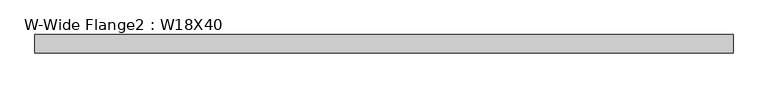
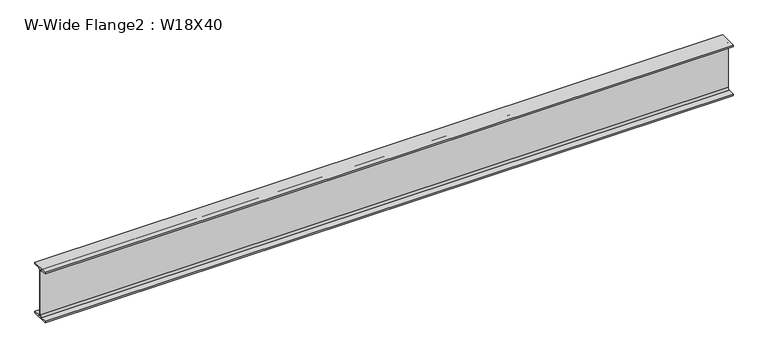
"""IFC4 building model written with IfcOpenShell, lengths in millimetres: beam geometry, W-Wide Flange2 : W18X40."""

from ifc_helpers import new_model, si_unit, point, frame, frame_2d, origin, place, context, project, spatial, polyline, circle_curve, trimmed, segment, composite_curve, outline, extrude, source, transform, mapped, element, save


def w_wide_flange2_w18x40_2cca02ce(model_context):
    return source(origin(), model_context, "Body", "SweptSolid", [
        extrude(outline(composite_curve([segment(polyline([(76.454, -213.995), (76.454, -227.33), (-76.454, -227.33), (-76.454, -213.995), (-20.828, -213.995)]), True, "CONTINUOUS"), segment(trimmed(circle_curve(frame_2d((-20.828, -197.1675)), 16.8275), [point((-20.828, -213.995))], [point((-4.0005, -197.1675))], True, "CARTESIAN"), True, "CONTINUOUS"), segment(polyline([(-4.0005, -197.1675), (-4.0005, 197.1675)]), True, "CONTINUOUS"), segment(trimmed(circle_curve(frame_2d((-20.828, 197.1675)), 16.8275), [point((-4.0005, 197.1675))], [point((-20.828, 213.995))], True, "CARTESIAN"), True, "CONTINUOUS"), segment(polyline([(-20.828, 213.995), (-76.454, 213.995), (-76.454, 227.33), (76.454, 227.33), (76.454, 213.995), (20.828, 213.995)]), True, "CONTINUOUS"), segment(trimmed(circle_curve(frame_2d((20.828, 197.1675)), 16.8275), [point((20.828, 213.995))], [point((4.0005, 197.1675))], True, "CARTESIAN"), True, "CONTINUOUS"), segment(polyline([(4.0005, 197.1675), (4.0005, -197.1675)]), True, "CONTINUOUS"), segment(trimmed(circle_curve(frame_2d((20.828, -197.1675)), 16.8275), [point((4.0005, -197.1675))], [point((20.828, -213.995))], True, "CARTESIAN"), True, "CONTINUOUS"), segment(polyline([(20.828, -213.995), (76.454, -213.995)]), True, "CONTINUOUS")], self_intersect=False)), frame((-2906.7125, 0.0, 0.0), z_axis=(1.0, 0.0, 0.0), x_axis=(0.0, 1.0, 0.0)), (0.0, 0.0, 1.0), 5870.575),
    ])


if __name__ == "__main__":
    model = new_model("IFC4")
    model_context = context("Model", 3, world=origin())
    ifc_project = project(units=[si_unit("LENGTHUNIT", "METRE", prefix="MILLI")], contexts=[model_context])
    site = spatial("IfcSite", under=ifc_project)
    building = spatial("IfcBuilding", under=site)
    placement = place(None, origin())
    w_wide_flange2_w18x40_shape = w_wide_flange2_w18x40_2cca02ce(model_context)
    element("IfcBeam", 1, ObjectType="W-Wide Flange2 : W18X40", at=placement, inside=building, context=model_context, shape_type="MappedRepresentation", body=[
        mapped(w_wide_flange2_w18x40_shape, transform((0.0, 0.0, 0.0), x_axis=(1.0, 0.0, 0.0), y_axis=(0.0, 1.0, 0.0), z_axis=(0.0, 0.0, 1.0))),
    ])
    save(model, "model.ifc")

# Revit data of these elements
# Type "W-Wide Flange2 : W18X40"
#   Assembly Code = "B10"
#   W = 40
#   Length [instance default] = 5' - 0"
#   bf = 0' - 6.02"
#   d = 1' - 5.9"
#   k = 0' - 1 3/16"
#   k2 = 0' - 0.6625"
#   tf = 0' - 0.525"
#   tw = 0' - 0.315"
#   A = 0.0819444 SF
#   Structural Material [instance default] = Steel ASTM A992
# Element 1 (IfcBeam, "W-Wide Flange2 : W18X40")
#   Materials on its faces: "Steel ASTM A992"
# Materials
#   "Steel ASTM A992": class "Metal", colour RGB 199 199 199, transparency 0, Description = "Structural steel 50ksi", Cost = 0
